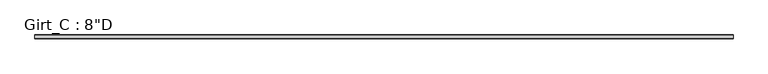
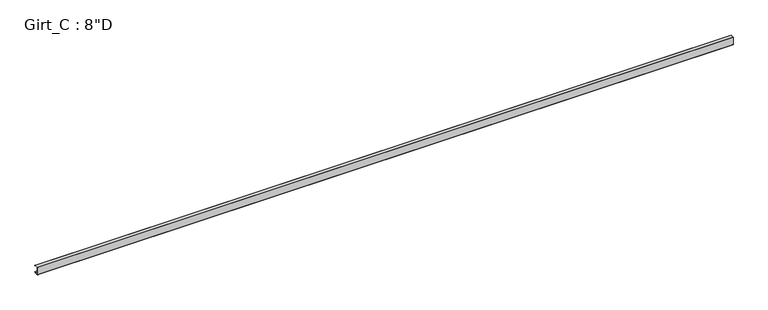
"""IFC4 building model written with IfcOpenShell, lengths in millimetres: beam geometry."""

from ifc_helpers import new_model, si_unit, point, frame, frame_2d, origin, place, context, project, spatial, polyline, circle_curve, trimmed, segment, composite_curve, outline, extrude, source, transform, mapped, element, save


def beam_b9b77de9(model_context):
    return source(origin(), model_context, "Body", "SweptSolid", [
        extrude(outline(composite_curve([segment(polyline([(87.5109375, 101.6), (99.7560415, 87.0068534), (97.6278742, 85.221109), (86.2154765, 98.821875), (3.3005807, 98.821875)]), True, "CONTINUOUS"), segment(trimmed(circle_curve(frame_2d((3.3741066, 96.8381931)), 1.9850441), [point((3.3005807, 98.821875))], [point((1.3890625, 96.8381931))], True, "CARTESIAN"), True, "CONTINUOUS"), segment(polyline([(1.3890625, 96.8381931), (1.3890625, -96.8389339)]), True, "CONTINUOUS"), segment(trimmed(circle_curve(frame_2d((3.3748024, -96.8389339)), 1.9857399), [point((1.3890625, -96.8389339))], [point((3.2694106, -98.821875))], True, "CARTESIAN"), True, "CONTINUOUS"), segment(polyline([(3.2694106, -98.821875), (86.2154765, -98.821875), (97.6510975, -85.1934327), (99.7792647, -86.979177), (87.5109375, -101.6), (3.3734375, -101.6)]), True, "CONTINUOUS"), segment(trimmed(circle_curve(frame_2d((3.3734375, -96.8375)), 4.7625), [point((3.3734375, -101.6))], [point((-1.3890625, -96.8375))], False, "CARTESIAN"), True, "CONTINUOUS"), segment(polyline([(-1.3890625, -96.8375), (-1.3890625, 96.8375)]), True, "CONTINUOUS"), segment(trimmed(circle_curve(frame_2d((3.3734375, 96.8375)), 4.7625), [point((-1.3890625, 96.8375))], [point((3.3734375, 101.6))], False, "CARTESIAN"), True, "CONTINUOUS"), segment(polyline([(3.3734375, 101.6), (87.5109375, 101.6)]), True, "CONTINUOUS")], self_intersect=False)), frame((-8812.2125, 0.0, 0.0), z_axis=(1.0, 0.0, 0.0), x_axis=(0.0, 1.0, 0.0)), (0.0, 0.0, 1.0), 17570.45),
    ])


if __name__ == "__main__":
    model = new_model("IFC4")
    model_context = context("Model", 3, world=origin())
    ifc_project = project(units=[si_unit("LENGTHUNIT", "METRE", prefix="MILLI")], contexts=[model_context])
    site = spatial("IfcSite", under=ifc_project)
    building = spatial("IfcBuilding", under=site)
    placement = place(None, origin())
    beam_shape = beam_b9b77de9(model_context)
    element("IfcBeam", 1, ObjectType="Girt_C : 8\"D", at=placement, inside=building, context=model_context, shape_type="MappedRepresentation", body=[
        mapped(beam_shape, transform((0.0, 0.0, 0.0), x_axis=(1.0, 0.0, 0.0), y_axis=(0.0, 1.0, 0.0), z_axis=(0.0, 0.0, 1.0))),
    ])
    save(model, "model.ifc")

# Revit data of these elements
# Type "Girt_C : 8\"D"
#   half leg = 0' - 1 3/4"
#   Web_Thickness = 0' - 0 7/64"
#   Length [instance default] = 10' - 0"
#   Leg_1 = 0' - 3 1/2"
#   Height = 0' - 8"
#   Structural Material [instance default] = none
# Element 1 (IfcBeam, "Girt_C : 8\"D")
#   Structural Material = CEE' SECTION (8.0x3.5C - SEE STRUCT. DWGS)
#   Materials on its faces: "CEE' SECTION (8.0x3.5C - SEE STRUCT. DWGS)"
# Materials
#   "CEE' SECTION (8.0x3.5C - SEE STRUCT. DWGS)": class "Metal", colour RGB 137 146 153, transparency 0, Description = "Steel, mill finish", Cost = 0
